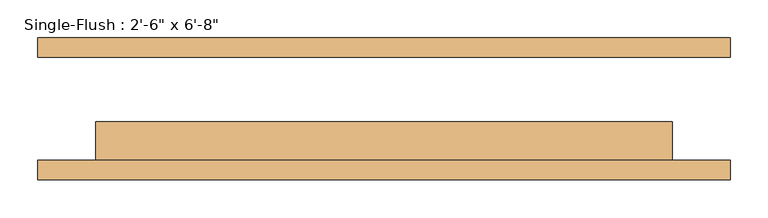
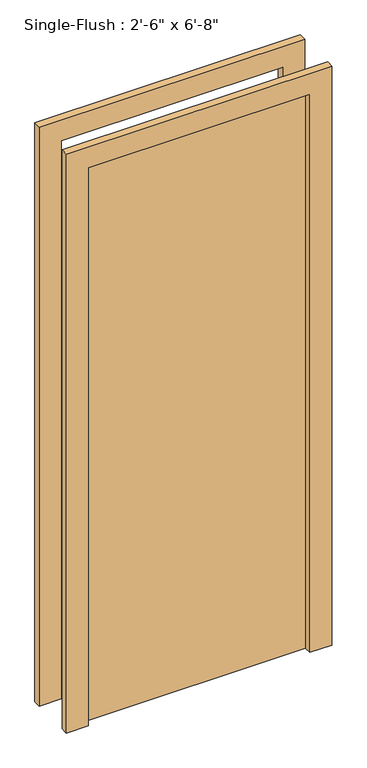
"""IFC4 building model written with IfcOpenShell, lengths in millimetres: door geometry."""

from ifc_helpers import new_model, si_unit, frame, origin, origin_with_axes, place, context, project, spatial, polyline, outline, extrude, source, transform, mapped, element, save


def door_cf295576(model_context):
    return source(origin(), model_context, "Body", "SweptSolid", [
        extrude(outline(polyline([(2108.2, -457.2), (0.0, -457.2), (0.0, -381.0), (2032.0, -381.0), (2032.0, 381.0), (0.0, 381.0), (0.0, 457.2), (2108.2, 457.2), (2108.2, -457.2)])), frame((0.0, -93.6625, 0.0), z_axis=(0.0, 1.0, 0.0), x_axis=(0.0, 0.0, 1.0)), (0.0, 0.0, 1.0), 25.4),
        extrude(outline(polyline([(2108.2, 457.2), (2108.2, -457.2), (0.0, -457.2), (0.0, -381.0), (2032.0, -381.0), (2032.0, 381.0), (0.0, 381.0), (0.0, 457.2), (2108.2, 457.2)])), frame((0.0, 68.2625, 0.0), z_axis=(0.0, 1.0, 0.0), x_axis=(0.0, 0.0, 1.0)), (0.0, 0.0, 1.0), 25.4),
        extrude(outline(polyline([(381.0, -17.4625), (381.0, -68.2625), (-381.0, -68.2625), (-381.0, -17.4625), (381.0, -17.4625)])), origin_with_axes(), (0.0, 0.0, 1.0), 2032.0),
    ])


if __name__ == "__main__":
    model = new_model("IFC4")
    model_context = context("Model", 3, world=origin())
    ifc_project = project(units=[si_unit("LENGTHUNIT", "METRE", prefix="MILLI")], contexts=[model_context])
    site = spatial("IfcSite", under=ifc_project)
    building = spatial("IfcBuilding", under=site)
    placement = place(None, origin())
    door_shape = door_cf295576(model_context)
    element("IfcDoor", 1, ObjectType="Single-Flush : 2'-6\" x 6'-8\"", at=placement, inside=building, context=model_context, shape_type="MappedRepresentation", body=[
        mapped(door_shape, transform((0.0, 0.0, 0.0), x_axis=(1.0, 0.0, 0.0), y_axis=(0.0, 1.0, 0.0), z_axis=(0.0, 0.0, 1.0))),
    ])
    save(model, "model.ifc")

# Revit data of these elements
# Type "Single-Flush : 2'-6\" x 6'-8\""
#   Type Mark = "13"
#   Construction Type Id = "MDOOR"
#   Assembly Code = "C1020"
#   Analytic Construction = "Metal"
#   Thickness = 0' - 2"
#   Heat Transfer Coefficient (U) = 3.7021 W/(m²·K)
#   Height = 6' - 8"
#   Trim Projection Ext = 0' - 1"
#   Trim Projection Int = 0' - 1"
#   Trim Width = 0' - 3"
#   Width = 2' - 6"
#   Door Material = Door - Panel
#   Frame Material = Door - Frame
#   Visual Light Transmittance = 0
#   Solar Heat Gain Coefficient = 0
#   Function = (empty or 0)
#   Wall Closure = (empty or 0)
# Element 1 (IfcDoor, "Single-Flush : 2'-6\" x 6'-8\"")
#   Materials on its faces: "Door - Frame", "Door - Panel"
# Materials
#   "Door - Panel": class "Wood", colour RGB 210 159 95, transparency 0, Cost = 0
#   "Door - Frame": class "Miscellaneous", colour RGB 118 70 51, transparency 0, Cost = 0
